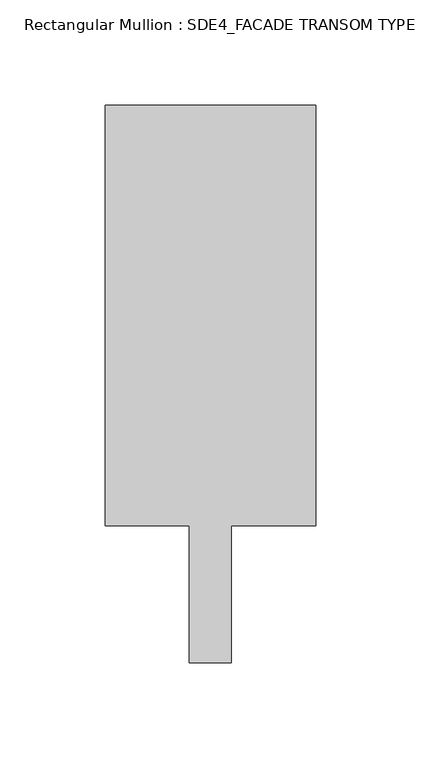
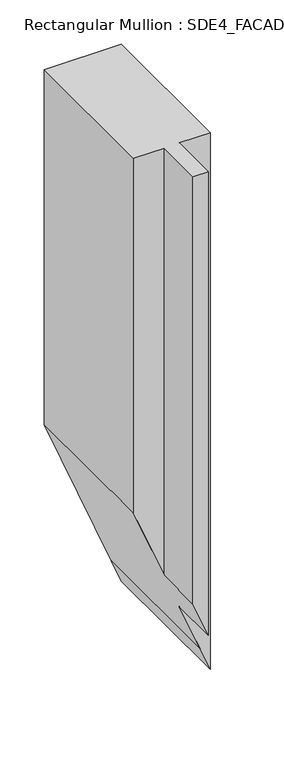
"""IFC4 building model written with IfcOpenShell, lengths in millimetres: member geometry, Rectangular Mullion : SDE4_FACADE TRANSOM TYPE 2."""

from ifc_helpers import new_model, si_unit, origin, place, context, project, spatial, faceted_brep, source, transform, mapped, element, save


def rectangular_mullion_sde4_facade_transom_type_2_87bea225(model_context):
    return source(origin(), model_context, "Body", "Brep", [
        faceted_brep([(50.0, 132.5, 0.0), (-50.0, 132.5, 0.0), (-50.0, -67.5, 0.0), (-10.0, -67.5, 0.0), (-10.0, -132.5, 0.0), (10.0, -132.5, 0.0), (10.0, -67.5, 0.0), (50.0, -67.5, 0.0), (50.0, 132.5, -737.2330639), (37.1390676, 132.5, -705.080733), (-50.0, 132.5, -487.2330639), (-50.0, -67.5, -487.2330639), (-10.0, -67.5, -587.2330639), (-10.0, -132.5, -587.2330639), (10.0, -132.5, -637.2330639), (10.0, -67.5, -637.2330639), (37.1390676, -67.5, -705.080733), (50.0, -67.5, -737.2330639)], [[[0, 1, 2, 3, 4, 5, 6, 7]], [[1, 0, 8, 9, 10]], [[2, 1, 10, 11]], [[3, 2, 11, 12]], [[4, 3, 12, 13]], [[5, 4, 13, 14]], [[6, 5, 14, 15]], [[7, 6, 15, 16, 17]], [[0, 7, 17, 8]], [[8, 17, 16, 9]], [[16, 15, 14, 13, 12, 11, 10, 9]]]),
    ])


if __name__ == "__main__":
    model = new_model("IFC4")
    model_context = context("Model", 3, world=origin())
    ifc_project = project(units=[si_unit("LENGTHUNIT", "METRE", prefix="MILLI")], contexts=[model_context])
    site = spatial("IfcSite", under=ifc_project)
    building = spatial("IfcBuilding", under=site)
    placement = place(None, origin())
    rectangular_mullion_sde4_facade_transom_type_2_shape = rectangular_mullion_sde4_facade_transom_type_2_87bea225(model_context)
    element("IfcMember", 1, ObjectType="Rectangular Mullion : SDE4_FACADE TRANSOM TYPE 2", at=placement, inside=building, context=model_context, shape_type="MappedRepresentation", body=[
        mapped(rectangular_mullion_sde4_facade_transom_type_2_shape, transform((0.0, 0.0, 0.0), x_axis=(1.0, 0.0, 0.0), y_axis=(0.0, 1.0, 0.0), z_axis=(0.0, 0.0, 1.0))),
    ])
    save(model, "model.ifc")

# Revit data of these elements
# Type "Rectangular Mullion : SDE4_FACADE TRANSOM TYPE 2"
#   built-in parameter 1007322 = 0.869423 (stored number, unit not read)
#   built-in parameter 1007321 = 0.164042 (stored number, unit not read)
#   built-in parameter 1007320 = 0.164042 (stored number, unit not read)
